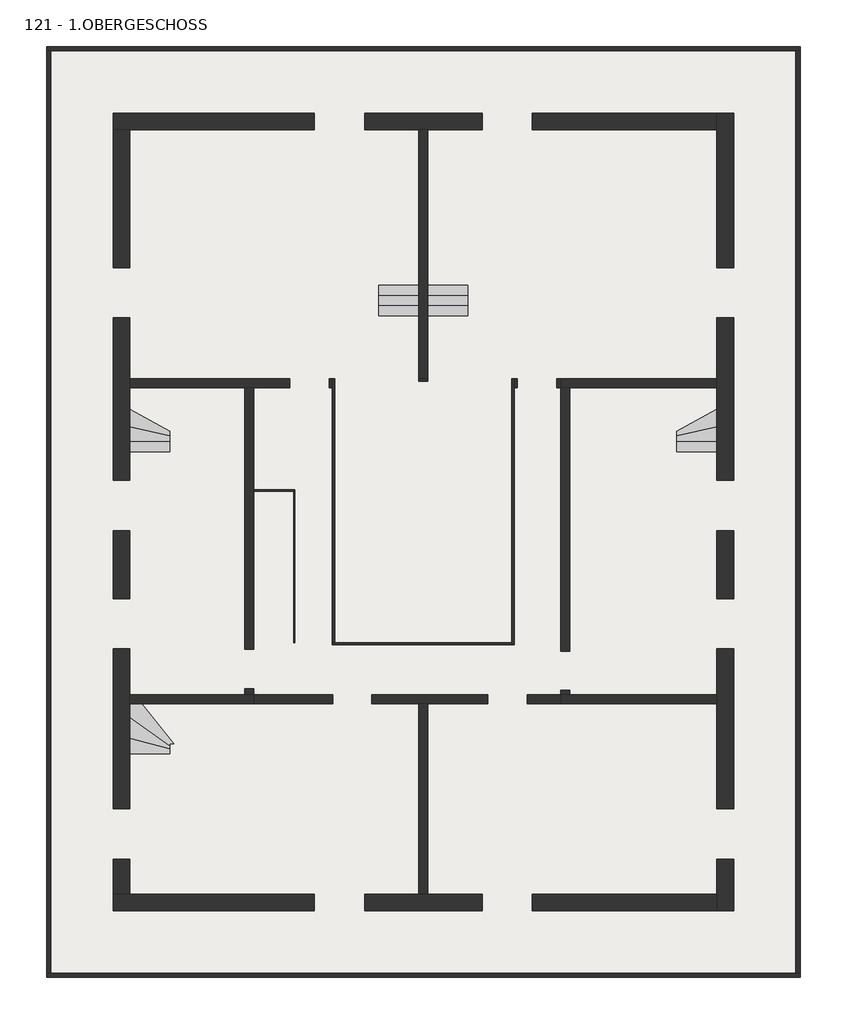
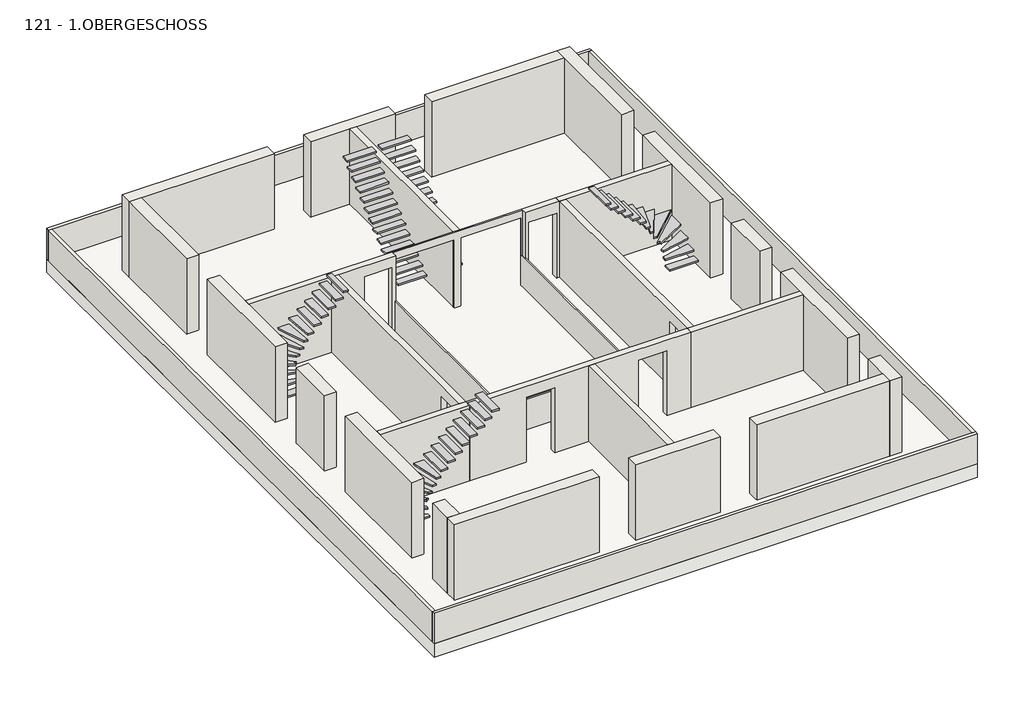
# One storey: 24 walls, 10 stairs, 1 slab.
# Revit data of these elements (continued)
# Project information
#   Organization Name = "Organization Name"
#   Organization Description = "Organization Description"
#   Building Name = "Building Name"
#   IfcOrganization = "KURIARCHITEKTEN"
#   IfcApplicationVersion = "2023.1"
#   IfcApplicationName = "Allplan"
#   IfcSite GUID = "3xMs$kp1n46ejeur8tozco"
#   IfcBuilding GUID = "0i8UyhEYT3nv9HLlo1H2X7"
#   IfcProject GUID = "2x1YFttxr4OvBiL8xtaqeA"
#   NameOverride = "GEBÄUDE 1"
#   Project Issue Date = "Issue Date"
#   Project Status = "Project Status"
#   Client Name = "Client Name"
#   Project Address = "Enter address here\nAddress Line 2"
#   Project Name = "Project Name"
#   Project Number = "Project Number"
# Type "Holzdecke 176 : Holzdecke 176"
#   Abrechnungsart = "m²"
#   Allright_Bauteil_ID = "0113De 0783954357"
#   Bezeichnung = "Holzdecke"
#   Codetext = "D-HOLZBALKEN1\\"
#   Gewerk = "Zimmer- und Holzbauarbeiten"
#   Material = "Holz"
#   Objektname = "Brettstapeldecke"
#   NameOverride = "Holzdecke"
#   Reference = "Holzdecke"
#   Status = "NEW"
#   PitchAngle = 0.00°
#   ThermalTransmittance = 0.0000 BTU/(h·ft²·°F)
#   2D Interaktion = yes
#   Combustible = no
#   Compartmentation = no
#   IsExternal = no
#   LoadBearing = yes
# Type "  97010 :   97010"
#   Abrechnungsart = "St"
#   Allright_Bauteil_ID = "0121Tre0785086959"
#   Material = "Stahlbeton"
#   Objektname = "Treppe"
#   NameOverride = " "
#   ThermalTransmittance = 0.0000 BTU/(h·ft²·°F)
#   NosingLength = 0.000 m
#   NumberOfRiser = 14
#   NumberOfTreads = 14
#   RiserHeight = 2.000 m
#   TreadLength = 2.300 m
#   IsExternal = no
#   FireExit = no
#   HandicapAccessible = no
#   HasNonSkidSurface = no
# Type "  97882 :   97882"
#   Abrechnungsart = "St"
#   Allright_Bauteil_ID = "0121Tre0785065280"
#   Codetext = "TR-MASSIV-GER\\"
#   Material = "Stahlbeton"
#   Objektname = "Treppe"
#   NameOverride = " "
#   Reference = "STB-Treppe"
#   ThermalTransmittance = 0.0000 BTU/(h·ft²·°F)
#   NosingLength = 0.000 m
#   NumberOfRiser = 14
#   NumberOfTreads = 13
#   RiserHeight = 2.021 m
#   TreadLength = 2.300 m
#   IsExternal = no
#   FireExit = no
#   HandicapAccessible = no
#   HasNonSkidSurface = no
# Type "  98300 :   98300"
#   Abrechnungsart = "St"
#   Allright_Bauteil_ID = "0121Tre0785065278"
#   Codetext = "TR-MASSIV-GER\\"
#   Material = "Stahlbeton"
#   Objektname = "Treppe"
#   NameOverride = " "
#   Reference = "STB-Treppe"
#   ThermalTransmittance = 0.0000 BTU/(h·ft²·°F)
#   NosingLength = 0.000 m
#   NumberOfRiser = 14
#   NumberOfTreads = 13
#   RiserHeight = 2.021 m
#   TreadLength = 2.300 m
#   IsExternal = no
#   FireExit = no
#   HandicapAccessible = no
#   HasNonSkidSurface = no
# Type "  98728 :   98728"
#   Abrechnungsart = "St"
#   Allright_Bauteil_ID = "0121Tre0785070507"
#   Material = "Stahlbeton"
#   Objektname = "Treppe"
#   NameOverride = " "
#   ThermalTransmittance = 0.0000 BTU/(h·ft²·°F)
#   NosingLength = 0.000 m
#   NumberOfRiser = 14
#   NumberOfTreads = 13
#   RiserHeight = 2.021 m
#   TreadLength = 2.300 m
#   IsExternal = no
#   FireExit = no
#   HandicapAccessible = no
#   HasNonSkidSurface = no
# Type "  99154 :   99154"
#   Abrechnungsart = "St"
#   Allright_Bauteil_ID = "0121Tre0785070829"
#   Material = "Stahlbeton"
#   Objektname = "Treppe"
#   NameOverride = " "
#   ThermalTransmittance = 0.0000 BTU/(h·ft²·°F)
#   NosingLength = 0.000 m
#   NumberOfRiser = 14
#   NumberOfTreads = 13
#   RiserHeight = 2.021 m
#   TreadLength = 2.300 m
#   IsExternal = no
#   FireExit = no
#   HandicapAccessible = no
#   HasNonSkidSurface = no
# Type "  149542 :   149542"
#   Abrechnungsart = "St"
#   Allright_Bauteil_ID = "0131Tre0659044515"
#   Material = "Stahlbeton"
#   Objektname = "Treppe"
#   NameOverride = " "
#   ThermalTransmittance = 0.0000 BTU/(h·ft²·°F)
#   NosingLength = 0.000 m
#   NumberOfRiser = 14
#   NumberOfTreads = 14
#   RiserHeight = 2.000 m
#   TreadLength = 2.300 m
#   IsExternal = no
#   FireExit = no
#   HandicapAccessible = no
#   HasNonSkidSurface = no
# Type "  150414 :   150414"
#   Abrechnungsart = "St"
#   Allright_Bauteil_ID = "0131Tre0659044575"
#   Codetext = "TR-MASSIV-GER\\"
#   Material = "Stahlbeton"
#   Objektname = "Treppe"
#   NameOverride = " "
#   Reference = "STB-Treppe"
#   ThermalTransmittance = 0.0000 BTU/(h·ft²·°F)
#   NosingLength = 0.000 m
#   NumberOfRiser = 14
#   NumberOfTreads = 13
#   RiserHeight = 2.021 m
#   TreadLength = 2.300 m
#   IsExternal = no
#   FireExit = no
#   HandicapAccessible = no
#   HasNonSkidSurface = no
# Type "  150832 :   150832"
#   Abrechnungsart = "St"
#   Allright_Bauteil_ID = "0131Tre0659044593"
#   Codetext = "TR-MASSIV-GER\\"
#   Material = "Stahlbeton"
#   Objektname = "Treppe"
#   NameOverride = " "
#   Reference = "STB-Treppe"
#   ThermalTransmittance = 0.0000 BTU/(h·ft²·°F)
#   NosingLength = 0.000 m
#   NumberOfRiser = 14
#   NumberOfTreads = 13
#   RiserHeight = 2.021 m
#   TreadLength = 2.300 m
#   IsExternal = no
#   FireExit = no
#   HandicapAccessible = no
#   HasNonSkidSurface = no
# Type "  151260 :   151260"
#   Abrechnungsart = "St"
#   Allright_Bauteil_ID = "0131Tre0659044533"
#   Material = "Stahlbeton"
#   Objektname = "Treppe"
#   NameOverride = " "
#   ThermalTransmittance = 0.0000 BTU/(h·ft²·°F)
#   NosingLength = 0.000 m
#   NumberOfRiser = 14
#   NumberOfTreads = 13
#   RiserHeight = 2.021 m
#   TreadLength = 2.300 m
#   IsExternal = no
#   FireExit = no
#   HandicapAccessible = no
#   HasNonSkidSurface = no
# Type "  151686 :   151686"
#   Abrechnungsart = "St"
#   Allright_Bauteil_ID = "0131Tre0659044570"
#   Material = "Stahlbeton"
#   Objektname = "Treppe"
#   NameOverride = " "
#   ThermalTransmittance = 0.0000 BTU/(h·ft²·°F)
#   NosingLength = 0.000 m
#   NumberOfRiser = 14
#   NumberOfTreads = 13
#   RiserHeight = 2.021 m
#   TreadLength = 2.300 m
#   IsExternal = no
#   FireExit = no
#   HandicapAccessible = no
#   HasNonSkidSurface = no
# Type " :1152"
#   Layers, outside or top first: 0.380 m "holzschalung" (function 1)
# Type " :1161"
#   Layers, outside or top first: 0.380 m "holzschalung" (function 1)
# Type " :1164"
#   Layers, outside or top first: 0.380 m "holzschalung" (function 1)
# Type " :1165"
#   Layers, outside or top first: 0.380 m "holzschalung" (function 1)
# Type " :1166"
#   Layers, outside or top first: 0.050 m "glas" (function 1)
# Type "Holzwand:1150"
#   ThermalTransmittance = 0.0000 BTU/(h·ft²·°F)
#   Combustible = no
#   Compartmentation = no
#   Layers, outside or top first: 0.200 m "holzschalung" (function 1)
# Type "Holzwand:1151"
#   ThermalTransmittance = 0.0000 BTU/(h·ft²·°F)
#   Combustible = no
#   Compartmentation = no
#   Layers, outside or top first: 0.200 m "holzschalung" (function 1)
# Type "Holzwand:1153"
#   ThermalTransmittance = 0.0000 BTU/(h·ft²·°F)
#   Combustible = no
#   Compartmentation = no
#   Layers, outside or top first: 0.200 m "holzschalung" (function 1)
# Type "Holzwand:1154"
#   ThermalTransmittance = 0.0000 BTU/(h·ft²·°F)
#   Combustible = no
#   Compartmentation = no
#   Layers, outside or top first: 0.030 m "holzschalung" (function 1)
# Type "Holzwand:1155"
#   ThermalTransmittance = 0.0000 BTU/(h·ft²·°F)
#   Combustible = no
#   Compartmentation = no
#   Layers, outside or top first: 0.030 m "holzschalung" (function 1)
# Type "Holzwand:1156"
#   ThermalTransmittance = 0.0000 BTU/(h·ft²·°F)
#   Combustible = no
#   Compartmentation = no
#   Layers, outside or top first: 0.200 m "holzschalung" (function 1)
# Type "Holzwand:1157"
#   ThermalTransmittance = 0.0000 BTU/(h·ft²·°F)
#   Combustible = no
#   Compartmentation = no
#   Layers, outside or top first: 0.200 m "holzschalung" (function 1)
# Type "Holzwand:1158"
#   ThermalTransmittance = 0.0000 BTU/(h·ft²·°F)
#   Combustible = no
#   Compartmentation = no
#   Layers, outside or top first: 0.200 m "holzschalung" (function 1)
# Type "Holzwand:1159"
#   ThermalTransmittance = 0.0000 BTU/(h·ft²·°F)
#   Combustible = no
#   Compartmentation = no
#   Layers, outside or top first: 0.200 m "holzschalung" (function 1)
# Type "Holzwand:1160"
#   ThermalTransmittance = 0.0000 BTU/(h·ft²·°F)
#   Combustible = no
#   Compartmentation = no
#   Layers, outside or top first: 0.200 m "holzschalung" (function 1)
# Type "Holzwand:1162"
#   ThermalTransmittance = 0.0000 BTU/(h·ft²·°F)
#   Combustible = no
#   Compartmentation = no
#   Layers, outside or top first: 0.200 m "holzschalung" (function 1)
# Type "Holzwand:1163"
#   ThermalTransmittance = 0.0000 BTU/(h·ft²·°F)
#   Combustible = no
#   Compartmentation = no
#   Layers, outside or top first: 0.200 m "holzschalung" (function 1)
# Type " :1167"
#   Layers, outside or top first: 0.050 m "holzschalung" (function 1)
# Type " :1168"
#   Layers, outside or top first: 0.050 m "holzschalung" (function 1)
# Type " :1169"
#   Layers, outside or top first: 0.050 m "holzschalung" (function 1)
# Type "Holzwand:1170"
#   ThermalTransmittance = 0.0000 BTU/(h·ft²·°F)
#   Combustible = no
#   Compartmentation = no
#   Layers, outside or top first: 0.100 m "pv - panel anthrazit" (function 1)
# Type "Holzwand:1171"
#   ThermalTransmittance = 0.0000 BTU/(h·ft²·°F)
#   Combustible = no
#   Compartmentation = no
#   Layers, outside or top first: 0.100 m "pv - panel anthrazit" (function 1)
# Type "Holzwand:1172"
#   ThermalTransmittance = 0.0000 BTU/(h·ft²·°F)
#   Combustible = no
#   Compartmentation = no
#   Layers, outside or top first: 0.100 m "pv - panel anthrazit" (function 1)
# Type "Holzwand:1173"
#   ThermalTransmittance = 0.0000 BTU/(h·ft²·°F)
#   Combustible = no
#   Compartmentation = no
#   Layers, outside or top first: 0.100 m "pv - panel anthrazit" (function 1)
# Element 1 (IfcSlab, "Holzdecke 176 : Holzdecke 176")
#   IFC Predefined Type = "FLOOR"
#   Export to IFC As = "ifcslab"
#   IfcGUID = "1_9Us2eVX4OuIZjhNyqdxW"
#   Phase Created = New Construction
#   Materials on its faces: "holzschalung"
# Element 2 (IfcStair, "  97010 :   97010")
#   IFC Predefined Type = "NOTDEFINED"
#   Export to IFC As = "ifcstair"
#   IfcGUID = "2ccaodaeb6QgHPV1d4NBnA"
#   Phase Created = New Construction
#   Materials on its faces: "weiss"
# Element 3 (IfcStair, "  97882 :   97882")
#   IFC Predefined Type = "STRAIGHT_RUN_STAIR"
#   Export to IFC As = "ifcstair"
#   IfcGUID = "1nghyUHoH9yBc_lxkBTUjw"
#   Phase Created = New Construction
#   Materials on its faces: "weiss"
# Element 4 (IfcStair, "  98300 :   98300")
#   IFC Predefined Type = "STRAIGHT_RUN_STAIR"
#   Export to IFC As = "ifcstair"
#   IfcGUID = "2AC_Gmfhz1LvYwUyPOxWan"
#   Phase Created = New Construction
#   Materials on its faces: "weiss"
# Element 5 (IfcStair, "  98728 :   98728")
#   IFC Predefined Type = "NOTDEFINED"
#   Export to IFC As = "ifcstair"
#   IfcGUID = "04Edcgbk9CPwWYiYhycXFf"
#   Phase Created = New Construction
#   Materials on its faces: "weiss"
# Element 6 (IfcStair, "  99154 :   99154")
#   IFC Predefined Type = "NOTDEFINED"
#   Export to IFC As = "ifcstair"
#   IfcGUID = "1azVXxNdn2POY9VYN93ccY"
#   Phase Created = New Construction
#   Materials on its faces: "weiss"
# Element 7 (IfcStair, "  149542 :   149542")
#   IFC Predefined Type = "NOTDEFINED"
#   Export to IFC As = "ifcstair"
#   IfcGUID = "1sH4rJKnLAFOtHPnXrLkif"
#   Phase Created = New Construction
#   Materials on its faces: "weiss"
# Element 8 (IfcStair, "  150414 :   150414")
#   IFC Predefined Type = "STRAIGHT_RUN_STAIR"
#   Export to IFC As = "ifcstair"
#   IfcGUID = "3fdccs_Mj1YAyFFpBc3gyk"
#   Phase Created = New Construction
#   Materials on its faces: "weiss"
# Element 9 (IfcStair, "  150832 :   150832")
#   IFC Predefined Type = "STRAIGHT_RUN_STAIR"
#   Export to IFC As = "ifcstair"
#   IfcGUID = "2szmEZdbD3KBDvfX1Sa6Vh"
#   Phase Created = New Construction
#   Materials on its faces: "weiss"
# Element 10 (IfcStair, "  151260 :   151260")
#   IFC Predefined Type = "NOTDEFINED"
#   Export to IFC As = "ifcstair"
#   IfcGUID = "1YKyaFTbr8YR41yGjubBsl"
#   Phase Created = New Construction
#   Materials on its faces: "weiss"
# Element 11 (IfcStair, "  151686 :   151686")
#   IFC Predefined Type = "NOTDEFINED"
#   Export to IFC As = "ifcstair"
#   IfcGUID = "2KPGRYHzzCygzBebAeLtPz"
#   Phase Created = New Construction
#   Materials on its faces: "weiss"
# Element 12 (IfcWall, " :1152")
#   Export to IFC As = "ifcwall"
#   IfcGUID = "2CeDj8YZTCPx$yj4WDVOez"
#   NameOverride = " "
#   Abrechnungsart = "m³"
#   Allright_Bauteil_ID = "0121HWa0785064286"
#   Layer #1:Object Layer Attributes #1:Abrechnungsart = "m²"
#   Layer #1:Object Layer Attributes #1:Allright_Bauteil_ID = "0121Wa 0785064367"
#   Layer #1:Object Layer Attributes #1:Gewerk = "Zimmer- und Holzbauarbeiten"
#   Layer #1:Object Layer Attributes #1:Material = "k.Ausw."
#   Layer #1:Object Layer Attributes #1:Objektname = "Wand"
#   Layer #1:Object Layer Attributes #1:Status = "Neubau"
#   MEP Wandtyp = "HO-WA-HSW\\"
#   Objektname = "Gesamtwand"
#   built-in parameter 1001111 = 0.505 m
#   Top Offset = 0.000 m
#   Base Offset = 0.505 m
#   Unconnected Height = 2.500 m
#   wall height = 2.500 m
#   Layer #1:Object Layer Attributes #1:2D Interaktion = yes
#   Phase Created = New Construction
#   Base Constraint = 121 - 1.OBERGESCHOSS
#   Materials on its faces: "holzschalung"
# Element 13 (IfcWall, " :1161")
#   Export to IFC As = "ifcwall"
#   IfcGUID = "2TnImcbz91shb3jN7Wgb8B"
#   NameOverride = " "
#   Abrechnungsart = "m³"
#   Allright_Bauteil_ID = "0121HWa0785064349"
#   Layer #1:Object Layer Attributes #1:Abrechnungsart = "m²"
#   Layer #1:Object Layer Attributes #1:Allright_Bauteil_ID = "0121Wa 0785064397"
#   Layer #1:Object Layer Attributes #1:Gewerk = "Zimmer- und Holzbauarbeiten"
#   Layer #1:Object Layer Attributes #1:Material = "k.Ausw."
#   Layer #1:Object Layer Attributes #1:Objektname = "Wand"
#   Layer #1:Object Layer Attributes #1:Status = "Neubau"
#   MEP Wandtyp = "HO-WA-HSW\\"
#   Objektname = "Gesamtwand"
#   built-in parameter 1001111 = 0.505 m
#   Top Offset = 0.000 m
#   Base Offset = 0.505 m
#   Unconnected Height = 2.500 m
#   wall height = 2.500 m
#   Layer #1:Object Layer Attributes #1:2D Interaktion = yes
#   Phase Created = New Construction
#   Base Constraint = 121 - 1.OBERGESCHOSS
#   Materials on its faces: "holzschalung"
# Element 14 (IfcWall, " :1164")
#   Export to IFC As = "ifcwall"
#   IfcGUID = "1tWRh4hxLAdASVw4VNE3to"
#   NameOverride = " "
#   Abrechnungsart = "m³"
#   Allright_Bauteil_ID = "0121HWa0785092952"
#   Layer #1:Object Layer Attributes #1:Abrechnungsart = "m²"
#   Layer #1:Object Layer Attributes #1:Allright_Bauteil_ID = "0121Wa 0785092986"
#   Layer #1:Object Layer Attributes #1:Gewerk = "Zimmer- und Holzbauarbeiten"
#   Layer #1:Object Layer Attributes #1:Material = "k.Ausw."
#   Layer #1:Object Layer Attributes #1:Objektname = "Wand"
#   Layer #1:Object Layer Attributes #1:Status = "Neubau"
#   MEP Wandtyp = "HO-WA-HSW\\"
#   Objektname = "Gesamtwand"
#   built-in parameter 1001111 = 0.505 m
#   Top Offset = 0.000 m
#   Base Offset = 0.505 m
#   Unconnected Height = 2.500 m
#   wall height = 2.500 m
#   Layer #1:Object Layer Attributes #1:2D Interaktion = yes
#   Phase Created = New Construction
#   Base Constraint = 121 - 1.OBERGESCHOSS
#   Materials on its faces: "holzschalung"
# Element 15 (IfcWall, " :1165")
#   Export to IFC As = "ifcwall"
#   IfcGUID = "1HE73MTmDEEBf4AV7ughZ8"
#   NameOverride = " "
#   Abrechnungsart = "m³"
#   Allright_Bauteil_ID = "0121HWa0785097898"
#   Layer #1:Object Layer Attributes #1:Abrechnungsart = "m²"
#   Layer #1:Object Layer Attributes #1:Allright_Bauteil_ID = "0121Wa 0785097934"
#   Layer #1:Object Layer Attributes #1:Gewerk = "Zimmer- und Holzbauarbeiten"
#   Layer #1:Object Layer Attributes #1:Material = "k.Ausw."
#   Layer #1:Object Layer Attributes #1:Objektname = "Wand"
#   Layer #1:Object Layer Attributes #1:Status = "Neubau"
#   MEP Wandtyp = "HO-WA-HSW\\"
#   Objektname = "Gesamtwand"
#   built-in parameter 1001111 = 0.505 m
#   Top Offset = 0.000 m
#   Base Offset = 0.505 m
#   Unconnected Height = 2.500 m
#   wall height = 2.500 m
#   Layer #1:Object Layer Attributes #1:2D Interaktion = yes
#   Phase Created = New Construction
#   Base Constraint = 121 - 1.OBERGESCHOSS
#   Materials on its faces: "holzschalung"
# Element 16 (IfcWall, " :1166")
#   Export to IFC As = "ifcwall"
#   IfcGUID = "0t2qqx1kvDZPNPdKl4bfzP"
#   NameOverride = " "
#   Abrechnungsart = "m³"
#   Allright_Bauteil_ID = "0121HWa0785064296"
#   Layer #1:Object Layer Attributes #1:Abrechnungsart = "m²"
#   Layer #1:Object Layer Attributes #1:Allright_Bauteil_ID = "0121Wa 0785064386"
#   Layer #1:Object Layer Attributes #1:Gewerk = "Zimmer- und Holzbauarbeiten"
#   Layer #1:Object Layer Attributes #1:Material = "k.Ausw."
#   Layer #1:Object Layer Attributes #1:Objektname = "Wand"
#   Layer #1:Object Layer Attributes #1:Status = "Neubau"
#   MEP Wandtyp = "HO-WA-HSW\\"
#   Objektname = "Gesamtwand"
#   built-in parameter 1001111 = 0.505 m
#   Top Offset = 0.000 m
#   Base Offset = 0.505 m
#   Unconnected Height = 2.500 m
#   wall height = 2.500 m
#   Layer #1:Object Layer Attributes #1:2D Interaktion = yes
#   Phase Created = New Construction
#   Base Constraint = 121 - 1.OBERGESCHOSS
#   Materials on its faces: "glas"
# Element 17 (IfcWall, "Holzwand:1150")
#   Export to IFC As = "ifcwall"
#   IfcGUID = "3nZ5Mon9nBjwoRgvyoor9a"
#   NameOverride = "Holzwand"
#   Abrechnungsart = "St"
#   Allright_Bauteil_ID = "0121HWa0785065367"
#   Bezeichnung = "Holzwand"
#   Layer #1:Object Layer Attributes #1:Abrechnungsart = "m²"
#   Layer #1:Object Layer Attributes #1:Allright_Bauteil_ID = "0121Wa 0785065369"
#   Layer #1:Object Layer Attributes #1:Bezeichnung = "Holzwand"
#   Layer #1:Object Layer Attributes #1:Codetext = "HO-WI-HSW\\"
#   Layer #1:Object Layer Attributes #1:Gewerk = "Zimmer- und Holzbauarbeiten"
#   Layer #1:Object Layer Attributes #1:Material = "Holz"
#   Layer #1:Object Layer Attributes #1:Objektname = "Wand"
#   Layer #1:Object Layer Attributes #1:Reference = "Holzwand"
#   Layer #1:Object Layer Attributes #1:Status = "Neubau"
#   MEP Wandtyp = "HO-WA-HSW\\"
#   Objektname = "Gesamtwand"
#   Reference = "Holzwand"
#   Status = "NEW"
#   built-in parameter 1001111 = 0.505 m
#   Top Offset = 0.000 m
#   Base Offset = 0.505 m
#   Unconnected Height = 2.500 m
#   wall height = 2.500 m
#   Layer #1:Object Layer Attributes #1:U-Wert = 0
#   Layer #1:Object Layer Attributes #1:2D Interaktion = yes
#   Layer #1:Object Layer Attributes #1:Außenbauteil = no
#   Layer #1:Object Layer Attributes #1:Brandabschnittsdefinierendes Bauteil = no
#   Layer #1:Object Layer Attributes #1:Brennbares Material = no
#   Layer #1:Object Layer Attributes #1:Raumhohe Wand = yes
#   Layer #1:Object Layer Attributes #1:Tragendes Bauteil = yes
#   ExtendToStructure = yes
#   IsExternal = no
#   LoadBearing = yes
#   Phase Created = New Construction
#   Base Constraint = 121 - 1.OBERGESCHOSS
#   Materials on its faces: "holzschalung"
# Element 18 (IfcWall, "Holzwand:1151")
#   Export to IFC As = "ifcwall"
#   IfcGUID = "3jE1E$NFj7vAP$vn70kdrt"
#   NameOverride = "Holzwand"
#   Abrechnungsart = "St"
#   Allright_Bauteil_ID = "0121HWa0785066899"
#   Bezeichnung = "Holzwand"
#   Layer #1:Object Layer Attributes #1:Abrechnungsart = "m²"
#   Layer #1:Object Layer Attributes #1:Allright_Bauteil_ID = "0121Wa 0785066901"
#   Layer #1:Object Layer Attributes #1:Bezeichnung = "Holzwand"
#   Layer #1:Object Layer Attributes #1:Codetext = "HO-WI-HSW\\"
#   Layer #1:Object Layer Attributes #1:Gewerk = "Zimmer- und Holzbauarbeiten"
#   Layer #1:Object Layer Attributes #1:Material = "Holz"
#   Layer #1:Object Layer Attributes #1:Objektname = "Wand"
#   Layer #1:Object Layer Attributes #1:Reference = "Holzwand"
#   Layer #1:Object Layer Attributes #1:Status = "Neubau"
#   MEP Wandtyp = "HO-WA-HSW\\"
#   Objektname = "Gesamtwand"
#   Reference = "Holzwand"
#   Status = "NEW"
#   built-in parameter 1001111 = 0.505 m
#   Top Offset = 0.000 m
#   Base Offset = 0.505 m
#   Unconnected Height = 2.500 m
#   wall height = 2.500 m
#   Layer #1:Object Layer Attributes #1:U-Wert = 0
#   Layer #1:Object Layer Attributes #1:2D Interaktion = yes
#   Layer #1:Object Layer Attributes #1:Außenbauteil = no
#   Layer #1:Object Layer Attributes #1:Brandabschnittsdefinierendes Bauteil = no
#   Layer #1:Object Layer Attributes #1:Brennbares Material = no
#   Layer #1:Object Layer Attributes #1:Raumhohe Wand = yes
#   Layer #1:Object Layer Attributes #1:Tragendes Bauteil = yes
#   ExtendToStructure = yes
#   IsExternal = no
#   LoadBearing = yes
#   Phase Created = New Construction
#   Base Constraint = 121 - 1.OBERGESCHOSS
#   Materials on its faces: "holzschalung"
# Element 19 (IfcWall, "Holzwand:1153")
#   Export to IFC As = "ifcwall"
#   IfcGUID = "1Zhxv5EALB9e6_$pCtUEXg"
#   NameOverride = "Holzwand"
#   Abrechnungsart = "St"
#   Allright_Bauteil_ID = "0121HWa0785065540"
#   Bezeichnung = "Holzwand"
#   Layer #1:Object Layer Attributes #1:Abrechnungsart = "m²"
#   Layer #1:Object Layer Attributes #1:Allright_Bauteil_ID = "0121Wa 0785065541"
#   Layer #1:Object Layer Attributes #1:Bezeichnung = "Holzwand"
#   Layer #1:Object Layer Attributes #1:Codetext = "HO-WI-HSW\\"
#   Layer #1:Object Layer Attributes #1:Gewerk = "Zimmer- und Holzbauarbeiten"
#   Layer #1:Object Layer Attributes #1:Material = "Holz"
#   Layer #1:Object Layer Attributes #1:Objektname = "Wand"
#   Layer #1:Object Layer Attributes #1:Reference = "Holzwand"
#   Layer #1:Object Layer Attributes #1:Status = "Neubau"
#   MEP Wandtyp = "HO-WA-HSW\\"
#   Objektname = "Gesamtwand"
#   Reference = "Holzwand"
#   Status = "NEW"
#   built-in parameter 1001111 = 0.505 m
#   Top Offset = 0.000 m
#   Base Offset = 0.505 m
#   Unconnected Height = 2.500 m
#   wall height = 2.500 m
#   Layer #1:Object Layer Attributes #1:U-Wert = 0
#   Layer #1:Object Layer Attributes #1:2D Interaktion = yes
#   Layer #1:Object Layer Attributes #1:Außenbauteil = no
#   Layer #1:Object Layer Attributes #1:Brandabschnittsdefinierendes Bauteil = no
#   Layer #1:Object Layer Attributes #1:Brennbares Material = no
#   Layer #1:Object Layer Attributes #1:Raumhohe Wand = yes
#   Layer #1:Object Layer Attributes #1:Tragendes Bauteil = yes
#   ExtendToStructure = yes
#   IsExternal = no
#   LoadBearing = yes
#   Phase Created = New Construction
#   Base Constraint = 121 - 1.OBERGESCHOSS
#   Materials on its faces: "holzschalung"
# Element 20 (IfcWall, "Holzwand:1154")
#   Export to IFC As = "ifcwall"
#   IfcGUID = "2MsVq3EJn0K8wHdQ6uoxnd"
#   NameOverride = "Holzwand"
#   Abrechnungsart = "St"
#   Allright_Bauteil_ID = "0121HWa0785067355"
#   Bezeichnung = "Holzwand"
#   Layer #1:Object Layer Attributes #1:Abrechnungsart = "m²"
#   Layer #1:Object Layer Attributes #1:Allright_Bauteil_ID = "0121Wa 0785067356"
#   Layer #1:Object Layer Attributes #1:Codetext = "HO-WI-HSW\\"
#   Layer #1:Object Layer Attributes #1:Gewerk = "Zimmer- und Holzbauarbeiten"
#   Layer #1:Object Layer Attributes #1:Material = "Holz"
#   Layer #1:Object Layer Attributes #1:Objektname = "Wand"
#   Layer #1:Object Layer Attributes #1:Reference = "Holzwand"
#   Layer #1:Object Layer Attributes #1:Status = "Neubau"
#   MEP Wandtyp = "HO-WA-HSW\\"
#   Objektname = "Gesamtwand"
#   Reference = "Holzwand"
#   Status = "NEW"
#   built-in parameter 1001111 = 0.505 m
#   Top Offset = 0.000 m
#   Base Offset = 0.505 m
#   Unconnected Height = 1.000 m
#   wall height = 1.000 m
#   Layer #1:Object Layer Attributes #1:U-Wert = 0
#   Layer #1:Object Layer Attributes #1:2D Interaktion = yes
#   Layer #1:Object Layer Attributes #1:Außenbauteil = no
#   Layer #1:Object Layer Attributes #1:Brandabschnittsdefinierendes Bauteil = no
#   Layer #1:Object Layer Attributes #1:Brennbares Material = no
#   Layer #1:Object Layer Attributes #1:Raumhohe Wand = yes
#   ExtendToStructure = yes
#   IsExternal = no
#   LoadBearing = yes
#   Phase Created = New Construction
#   Base Constraint = 121 - 1.OBERGESCHOSS
#   Materials on its faces: "holzschalung"
# Element 21 (IfcWall, "Holzwand:1155")
#   Export to IFC As = "ifcwall"
#   IfcGUID = "1F_ySrDsP9oP3MqXymSTVO"
#   NameOverride = "Holzwand"
#   Abrechnungsart = "St"
#   Allright_Bauteil_ID = "0121HWa0785067347"
#   Bezeichnung = "Holzwand"
#   Layer #1:Object Layer Attributes #1:Abrechnungsart = "m²"
#   Layer #1:Object Layer Attributes #1:Allright_Bauteil_ID = "0121Wa 0785067348"
#   Layer #1:Object Layer Attributes #1:Codetext = "HO-WI-HSW\\"
#   Layer #1:Object Layer Attributes #1:Gewerk = "Zimmer- und Holzbauarbeiten"
#   Layer #1:Object Layer Attributes #1:Material = "Holz"
#   Layer #1:Object Layer Attributes #1:Objektname = "Wand"
#   Layer #1:Object Layer Attributes #1:Reference = "Holzwand"
#   Layer #1:Object Layer Attributes #1:Status = "Neubau"
#   MEP Wandtyp = "HO-WA-HSW\\"
#   Objektname = "Gesamtwand"
#   Reference = "Holzwand"
#   Status = "NEW"
#   built-in parameter 1001111 = 0.505 m
#   Top Offset = 0.000 m
#   Base Offset = 0.505 m
#   Unconnected Height = 1.000 m
#   wall height = 1.000 m
#   Layer #1:Object Layer Attributes #1:U-Wert = 0
#   Layer #1:Object Layer Attributes #1:2D Interaktion = yes
#   Layer #1:Object Layer Attributes #1:Außenbauteil = no
#   Layer #1:Object Layer Attributes #1:Brandabschnittsdefinierendes Bauteil = no
#   Layer #1:Object Layer Attributes #1:Brennbares Material = no
#   Layer #1:Object Layer Attributes #1:Raumhohe Wand = yes
#   ExtendToStructure = yes
#   IsExternal = no
#   LoadBearing = yes
#   Phase Created = New Construction
#   Base Constraint = 121 - 1.OBERGESCHOSS
#   Materials on its faces: "holzschalung"
# Element 22 (IfcWall, "Holzwand:1156")
#   Export to IFC As = "ifcwall"
#   IfcGUID = "0gtwZwppj1pObqyI7HY41_"
#   NameOverride = "Holzwand"
#   Abrechnungsart = "St"
#   Allright_Bauteil_ID = "0121HWa0785064323"
#   Bezeichnung = "Holzwand"
#   Layer #1:Object Layer Attributes #1:Abrechnungsart = "m²"
#   Layer #1:Object Layer Attributes #1:Allright_Bauteil_ID = "0121Wa 0785064369"
#   Layer #1:Object Layer Attributes #1:Bezeichnung = "Holzwand"
#   Layer #1:Object Layer Attributes #1:Codetext = "HO-WI-HSW\\"
#   Layer #1:Object Layer Attributes #1:Gewerk = "Zimmer- und Holzbauarbeiten"
#   Layer #1:Object Layer Attributes #1:Material = "Holz"
#   Layer #1:Object Layer Attributes #1:Objektname = "Wand"
#   Layer #1:Object Layer Attributes #1:Reference = "Holzwand"
#   Layer #1:Object Layer Attributes #1:Status = "Neubau"
#   MEP Wandtyp = "HO-WA-HSW\\"
#   Objektname = "Gesamtwand"
#   Reference = "Holzwand"
#   Status = "NEW"
#   built-in parameter 1001111 = 0.505 m
#   Top Offset = 0.000 m
#   Base Offset = 0.505 m
#   Unconnected Height = 2.500 m
#   wall height = 2.500 m
#   Layer #1:Object Layer Attributes #1:U-Wert = 0
#   Layer #1:Object Layer Attributes #1:2D Interaktion = yes
#   Layer #1:Object Layer Attributes #1:Außenbauteil = no
#   Layer #1:Object Layer Attributes #1:Brandabschnittsdefinierendes Bauteil = no
#   Layer #1:Object Layer Attributes #1:Brennbares Material = no
#   Layer #1:Object Layer Attributes #1:Raumhohe Wand = yes
#   Layer #1:Object Layer Attributes #1:Tragendes Bauteil = yes
#   ExtendToStructure = yes
#   IsExternal = no
#   LoadBearing = yes
#   Phase Created = New Construction
#   Base Constraint = 121 - 1.OBERGESCHOSS
#   Materials on its faces: "holzschalung"
# Element 23 (IfcWall, "Holzwand:1157")
#   Export to IFC As = "ifcwall"
#   IfcGUID = "0tY6$O1l121AktLhYSWZjf"
#   NameOverride = "Holzwand"
#   Abrechnungsart = "St"
#   Allright_Bauteil_ID = "0121HWa0785064381"
#   Bezeichnung = "Holzwand"
#   Layer #1:Object Layer Attributes #1:Abrechnungsart = "m²"
#   Layer #1:Object Layer Attributes #1:Allright_Bauteil_ID = "0121Wa 0785064384"
#   Layer #1:Object Layer Attributes #1:Bezeichnung = "Holzwand"
#   Layer #1:Object Layer Attributes #1:Codetext = "HO-WI-HSW\\"
#   Layer #1:Object Layer Attributes #1:Gewerk = "Zimmer- und Holzbauarbeiten"
#   Layer #1:Object Layer Attributes #1:Material = "Holz"
#   Layer #1:Object Layer Attributes #1:Objektname = "Wand"
#   Layer #1:Object Layer Attributes #1:Reference = "Holzwand"
#   Layer #1:Object Layer Attributes #1:Status = "Neubau"
#   MEP Wandtyp = "HO-WA-HSW\\"
#   Objektname = "Gesamtwand"
#   Reference = "Holzwand"
#   Status = "NEW"
#   built-in parameter 1001111 = 0.505 m
#   Top Offset = 0.000 m
#   Base Offset = 0.505 m
#   Unconnected Height = 2.500 m
#   wall height = 2.500 m
#   Layer #1:Object Layer Attributes #1:U-Wert = 0
#   Layer #1:Object Layer Attributes #1:2D Interaktion = yes
#   Layer #1:Object Layer Attributes #1:Außenbauteil = no
#   Layer #1:Object Layer Attributes #1:Brandabschnittsdefinierendes Bauteil = no
#   Layer #1:Object Layer Attributes #1:Brennbares Material = no
#   Layer #1:Object Layer Attributes #1:Raumhohe Wand = yes
#   Layer #1:Object Layer Attributes #1:Tragendes Bauteil = yes
#   ExtendToStructure = yes
#   IsExternal = no
#   LoadBearing = yes
#   Phase Created = New Construction
#   Base Constraint = 121 - 1.OBERGESCHOSS
#   Materials on its faces: "holzschalung"
# Element 24 (IfcWall, "Holzwand:1158")
#   Export to IFC As = "ifcwall"
#   IfcGUID = "2Mr8L52dj4iP8MoJTiOa9p"
#   NameOverride = "Holzwand"
#   Abrechnungsart = "St"
#   Allright_Bauteil_ID = "0121HWa0785069286"
#   Bezeichnung = "Holzwand"
#   Layer #1:Object Layer Attributes #1:Abrechnungsart = "m²"
#   Layer #1:Object Layer Attributes #1:Allright_Bauteil_ID = "0121Wa 0785069294"
#   Layer #1:Object Layer Attributes #1:Bezeichnung = "Holzwand"
#   Layer #1:Object Layer Attributes #1:Codetext = "HO-WI-HSW\\"
#   Layer #1:Object Layer Attributes #1:Gewerk = "Zimmer- und Holzbauarbeiten"
#   Layer #1:Object Layer Attributes #1:Material = "Holz"
#   Layer #1:Object Layer Attributes #1:Objektname = "Wand"
#   Layer #1:Object Layer Attributes #1:Reference = "Holzwand"
#   Layer #1:Object Layer Attributes #1:Status = "Neubau"
#   MEP Wandtyp = "HO-WA-HSW\\"
#   Objektname = "Gesamtwand"
#   Reference = "Holzwand"
#   Status = "NEW"
#   built-in parameter 1001111 = 0.505 m
#   Top Offset = 0.000 m
#   Base Offset = 0.505 m
#   Unconnected Height = 2.500 m
#   wall height = 2.500 m
#   Layer #1:Object Layer Attributes #1:U-Wert = 0
#   Layer #1:Object Layer Attributes #1:2D Interaktion = yes
#   Layer #1:Object Layer Attributes #1:Außenbauteil = no
#   Layer #1:Object Layer Attributes #1:Brandabschnittsdefinierendes Bauteil = no
#   Layer #1:Object Layer Attributes #1:Brennbares Material = no
#   Layer #1:Object Layer Attributes #1:Raumhohe Wand = yes
#   Layer #1:Object Layer Attributes #1:Tragendes Bauteil = yes
#   ExtendToStructure = yes
#   IsExternal = no
#   LoadBearing = yes
#   Phase Created = New Construction
#   Base Constraint = 121 - 1.OBERGESCHOSS
#   Materials on its faces: "holzschalung"
# Element 25 (IfcWall, "Holzwand:1159")
#   Export to IFC As = "ifcwall"
#   IfcGUID = "36leNf4gL9OB_v358ffY76"
#   NameOverride = "Holzwand"
#   Abrechnungsart = "St"
#   Allright_Bauteil_ID = "0121HWa0785064324"
#   Bezeichnung = "Holzwand"
#   Layer #1:Object Layer Attributes #1:Abrechnungsart = "m²"
#   Layer #1:Object Layer Attributes #1:Allright_Bauteil_ID = "0121Wa 0785064395"
#   Layer #1:Object Layer Attributes #1:Bezeichnung = "Holzwand"
#   Layer #1:Object Layer Attributes #1:Codetext = "HO-WI-HSW\\"
#   Layer #1:Object Layer Attributes #1:Gewerk = "Zimmer- und Holzbauarbeiten"
#   Layer #1:Object Layer Attributes #1:Material = "Holz"
#   Layer #1:Object Layer Attributes #1:Objektname = "Wand"
#   Layer #1:Object Layer Attributes #1:Reference = "Holzwand"
#   Layer #1:Object Layer Attributes #1:Status = "Neubau"
#   MEP Wandtyp = "HO-WA-HSW\\"
#   Objektname = "Gesamtwand"
#   Reference = "Holzwand"
#   Status = "NEW"
#   built-in parameter 1001111 = 0.505 m
#   Top Offset = 0.000 m
#   Base Offset = 0.505 m
#   Unconnected Height = 2.500 m
#   wall height = 2.500 m
#   Layer #1:Object Layer Attributes #1:U-Wert = 0
#   Layer #1:Object Layer Attributes #1:2D Interaktion = yes
#   Layer #1:Object Layer Attributes #1:Außenbauteil = no
#   Layer #1:Object Layer Attributes #1:Brandabschnittsdefinierendes Bauteil = no
#   Layer #1:Object Layer Attributes #1:Brennbares Material = no
#   Layer #1:Object Layer Attributes #1:Raumhohe Wand = yes
#   Layer #1:Object Layer Attributes #1:Tragendes Bauteil = yes
#   ExtendToStructure = yes
#   IsExternal = no
#   LoadBearing = yes
#   Phase Created = New Construction
#   Base Constraint = 121 - 1.OBERGESCHOSS
#   Materials on its faces: "holzschalung"
# Element 26 (IfcWall, "Holzwand:1160")
#   Export to IFC As = "ifcwall"
#   IfcGUID = "3kHHpx_NTE_9JnfL3dFkYB"
#   NameOverride = "Holzwand"
#   Abrechnungsart = "St"
#   Allright_Bauteil_ID = "0121HWa0785064389"
#   Bezeichnung = "Holzwand"
#   Layer #1:Object Layer Attributes #1:Abrechnungsart = "m²"
#   Layer #1:Object Layer Attributes #1:Allright_Bauteil_ID = "0121Wa 0785064393"
#   Layer #1:Object Layer Attributes #1:Bezeichnung = "Holzwand"
#   Layer #1:Object Layer Attributes #1:Codetext = "HO-WI-HSW\\"
#   Layer #1:Object Layer Attributes #1:Gewerk = "Zimmer- und Holzbauarbeiten"
#   Layer #1:Object Layer Attributes #1:Material = "Holz"
#   Layer #1:Object Layer Attributes #1:Objektname = "Wand"
#   Layer #1:Object Layer Attributes #1:Reference = "Holzwand"
#   Layer #1:Object Layer Attributes #1:Status = "Neubau"
#   MEP Wandtyp = "HO-WA-HSW\\"
#   Objektname = "Gesamtwand"
#   Reference = "Holzwand"
#   Status = "NEW"
#   built-in parameter 1001111 = 0.505 m
#   Top Offset = 0.000 m
#   Base Offset = 0.505 m
#   Unconnected Height = 2.500 m
#   wall height = 2.500 m
#   Layer #1:Object Layer Attributes #1:U-Wert = 0
#   Layer #1:Object Layer Attributes #1:2D Interaktion = yes
#   Layer #1:Object Layer Attributes #1:Außenbauteil = no
#   Layer #1:Object Layer Attributes #1:Brandabschnittsdefinierendes Bauteil = no
#   Layer #1:Object Layer Attributes #1:Brennbares Material = no
#   Layer #1:Object Layer Attributes #1:Raumhohe Wand = yes
#   Layer #1:Object Layer Attributes #1:Tragendes Bauteil = yes
#   ExtendToStructure = yes
#   IsExternal = no
#   LoadBearing = yes
#   Phase Created = New Construction
#   Base Constraint = 121 - 1.OBERGESCHOSS
#   Materials on its faces: "holzschalung"
# Element 27 (IfcWall, "Holzwand:1162")
#   Export to IFC As = "ifcwall"
#   IfcGUID = "26lQuimMP00PZvPhbBRI2R"
#   NameOverride = "Holzwand"
#   Abrechnungsart = "St"
#   Allright_Bauteil_ID = "0121HWa0785065329"
#   Bezeichnung = "Holzwand"
#   Layer #1:Object Layer Attributes #1:Abrechnungsart = "m²"
#   Layer #1:Object Layer Attributes #1:Allright_Bauteil_ID = "0121Wa 0785065331"
#   Layer #1:Object Layer Attributes #1:Bezeichnung = "Holzwand"
#   Layer #1:Object Layer Attributes #1:Codetext = "HO-WI-HSW\\"
#   Layer #1:Object Layer Attributes #1:Gewerk = "Zimmer- und Holzbauarbeiten"
#   Layer #1:Object Layer Attributes #1:Material = "Holz"
#   Layer #1:Object Layer Attributes #1:Objektname = "Wand"
#   Layer #1:Object Layer Attributes #1:Reference = "Holzwand"
#   Layer #1:Object Layer Attributes #1:Status = "Neubau"
#   MEP Wandtyp = "HO-WA-HSW\\"
#   Objektname = "Gesamtwand"
#   Reference = "Holzwand"
#   Status = "NEW"
#   built-in parameter 1001111 = 0.505 m
#   Top Offset = 0.000 m
#   Base Offset = 0.505 m
#   Unconnected Height = 2.500 m
#   wall height = 2.500 m
#   Layer #1:Object Layer Attributes #1:U-Wert = 0
#   Layer #1:Object Layer Attributes #1:2D Interaktion = yes
#   Layer #1:Object Layer Attributes #1:Außenbauteil = no
#   Layer #1:Object Layer Attributes #1:Brandabschnittsdefinierendes Bauteil = no
#   Layer #1:Object Layer Attributes #1:Brennbares Material = no
#   Layer #1:Object Layer Attributes #1:Raumhohe Wand = yes
#   Layer #1:Object Layer Attributes #1:Tragendes Bauteil = yes
#   ExtendToStructure = yes
#   IsExternal = no
#   LoadBearing = yes
#   Phase Created = New Construction
#   Base Constraint = 121 - 1.OBERGESCHOSS
#   Materials on its faces: "holzschalung"
# Element 28 (IfcWall, "Holzwand:1163")
#   Export to IFC As = "ifcwall"
#   IfcGUID = "3atU$IMTH8YP$GZozT8ehc"
#   NameOverride = "Holzwand"
#   Abrechnungsart = "St"
#   Allright_Bauteil_ID = "0121HWa0785064334"
#   Bezeichnung = "Holzwand"
#   Layer #1:Object Layer Attributes #1:Abrechnungsart = "m²"
#   Layer #1:Object Layer Attributes #1:Allright_Bauteil_ID = "0121Wa 0785064371"
#   Layer #1:Object Layer Attributes #1:Bezeichnung = "Holzwand"
#   Layer #1:Object Layer Attributes #1:Codetext = "HO-WI-HSW\\"
#   Layer #1:Object Layer Attributes #1:Gewerk = "Zimmer- und Holzbauarbeiten"
#   Layer #1:Object Layer Attributes #1:Material = "Holz"
#   Layer #1:Object Layer Attributes #1:Objektname = "Wand"
#   Layer #1:Object Layer Attributes #1:Reference = "Holzwand"
#   Layer #1:Object Layer Attributes #1:Status = "Neubau"
#   MEP Wandtyp = "HO-WA-HSW\\"
#   Objektname = "Gesamtwand"
#   Reference = "Holzwand"
#   Status = "NEW"
#   built-in parameter 1001111 = 0.505 m
#   Top Offset = 0.000 m
#   Base Offset = 0.505 m
#   Unconnected Height = 2.500 m
#   wall height = 2.500 m
#   Layer #1:Object Layer Attributes #1:U-Wert = 0
#   Layer #1:Object Layer Attributes #1:2D Interaktion = yes
#   Layer #1:Object Layer Attributes #1:Außenbauteil = no
#   Layer #1:Object Layer Attributes #1:Brandabschnittsdefinierendes Bauteil = no
#   Layer #1:Object Layer Attributes #1:Brennbares Material = no
#   Layer #1:Object Layer Attributes #1:Raumhohe Wand = yes
#   Layer #1:Object Layer Attributes #1:Tragendes Bauteil = yes
#   ExtendToStructure = yes
#   IsExternal = no
#   LoadBearing = yes
#   Phase Created = New Construction
#   Base Constraint = 121 - 1.OBERGESCHOSS
#   Materials on its faces: "holzschalung"
# Element 29 (IfcWall, " :1167")
#   Export to IFC As = "ifcwall"
#   IfcGUID = "35Iolt9MTFw82QPYPk5JvU"
#   NameOverride = " "
#   Abrechnungsart = "m³"
#   Allright_Bauteil_ID = "0121HWa0785064294"
#   Layer #1:Object Layer Attributes #1:Abrechnungsart = "m²"
#   Layer #1:Object Layer Attributes #1:Allright_Bauteil_ID = "0121Wa 0785064340"
#   Layer #1:Object Layer Attributes #1:Gewerk = "Zimmer- und Holzbauarbeiten"
#   Layer #1:Object Layer Attributes #1:Material = "k.Ausw."
#   Layer #1:Object Layer Attributes #1:Objektname = "Wand"
#   Layer #1:Object Layer Attributes #1:Status = "Neubau"
#   MEP Wandtyp = "HO-WA-HSW\\"
#   Objektname = "Gesamtwand"
#   built-in parameter 1001111 = 0.505 m
#   Top Offset = 0.000 m
#   Base Offset = 0.505 m
#   Unconnected Height = 1.000 m
#   wall height = 1.000 m
#   Layer #1:Object Layer Attributes #1:2D Interaktion = yes
#   Layer #1:Object Layer Attributes #1:Tragendes Bauteil = no
#   Phase Created = New Construction
#   Base Constraint = 121 - 1.OBERGESCHOSS
#   Materials on its faces: "holzschalung", "glas"
# Element 30 (IfcWall, " :1168")
#   Export to IFC As = "ifcwall"
#   IfcGUID = "21NDiotIv7sAO2c5Bbio25"
#   NameOverride = " "
#   Abrechnungsart = "m³"
#   Allright_Bauteil_ID = "0121HWa0785064290"
#   Layer #1:Object Layer Attributes #1:Abrechnungsart = "m²"
#   Layer #1:Object Layer Attributes #1:Allright_Bauteil_ID = "0121Wa 0785064348"
#   Layer #1:Object Layer Attributes #1:Gewerk = "Zimmer- und Holzbauarbeiten"
#   Layer #1:Object Layer Attributes #1:Material = "k.Ausw."
#   Layer #1:Object Layer Attributes #1:Objektname = "Wand"
#   Layer #1:Object Layer Attributes #1:Status = "Neubau"
#   MEP Wandtyp = "HO-WA-HSW\\"
#   Objektname = "Gesamtwand"
#   built-in parameter 1001111 = 0.505 m
#   Top Offset = 0.000 m
#   Base Offset = 0.505 m
#   Unconnected Height = 1.000 m
#   wall height = 1.000 m
#   Layer #1:Object Layer Attributes #1:2D Interaktion = yes
#   Layer #1:Object Layer Attributes #1:Tragendes Bauteil = no
#   Phase Created = New Construction
#   Base Constraint = 121 - 1.OBERGESCHOSS
#   Materials on its faces: "holzschalung"
# Element 31 (IfcWall, " :1169")
#   Export to IFC As = "ifcwall"
#   IfcGUID = "2aL_F8tebFMgUeEEKPH5KO"
#   NameOverride = " "
#   Abrechnungsart = "m³"
#   Allright_Bauteil_ID = "0121HWa0785064292"
#   Layer #1:Object Layer Attributes #1:Abrechnungsart = "m²"
#   Layer #1:Object Layer Attributes #1:Allright_Bauteil_ID = "0121Wa 0785064346"
#   Layer #1:Object Layer Attributes #1:Gewerk = "Zimmer- und Holzbauarbeiten"
#   Layer #1:Object Layer Attributes #1:Material = "k.Ausw."
#   Layer #1:Object Layer Attributes #1:Objektname = "Wand"
#   Layer #1:Object Layer Attributes #1:Status = "Neubau"
#   MEP Wandtyp = "HO-WA-HSW\\"
#   Objektname = "Gesamtwand"
#   built-in parameter 1001111 = 0.505 m
#   Top Offset = 0.000 m
#   Base Offset = 0.505 m
#   Unconnected Height = 1.000 m
#   wall height = 1.000 m
#   Layer #1:Object Layer Attributes #1:2D Interaktion = yes
#   Layer #1:Object Layer Attributes #1:Tragendes Bauteil = no
#   Phase Created = New Construction
#   Base Constraint = 121 - 1.OBERGESCHOSS
#   Materials on its faces: "holzschalung", "glas"
# Element 32 (IfcWall, "Holzwand:1170")
#   Export to IFC As = "ifcwall"
#   IfcGUID = "2$ckBCNA58Zga6x6IbH4cF"
#   NameOverride = "Holzwand"
#   Abrechnungsart = "St"
#   Allright_Bauteil_ID = "0127HWa0783955754"
#   Bezeichnung = "Holzwand"
#   Layer #1:Object Layer Attributes #1:Abrechnungsart = "m²"
#   Layer #1:Object Layer Attributes #1:Allright_Bauteil_ID = "0127Wa 0783955755"
#   Layer #1:Object Layer Attributes #1:Codetext = "HO-WI-HSW\\"
#   Layer #1:Object Layer Attributes #1:Gewerk = "Zimmer- und Holzbauarbeiten"
#   Layer #1:Object Layer Attributes #1:Material = "Holz"
#   Layer #1:Object Layer Attributes #1:Objektname = "Wand"
#   Layer #1:Object Layer Attributes #1:Reference = "Holzwand"
#   Layer #1:Object Layer Attributes #1:Status = "Neubau"
#   MEP Wandtyp = "HO-WA-HSW\\"
#   Objektname = "Gesamtwand"
#   Reference = "Holzwand"
#   Status = "NEW"
#   built-in parameter 1001111 = 0.505 m
#   Top Offset = 0.000 m
#   Base Offset = 0.505 m
#   Unconnected Height = 1.000 m
#   wall height = 1.000 m
#   Layer #1:Object Layer Attributes #1:U-Wert = 0
#   Layer #1:Object Layer Attributes #1:2D Interaktion = yes
#   Layer #1:Object Layer Attributes #1:Außenbauteil = no
#   Layer #1:Object Layer Attributes #1:Brandabschnittsdefinierendes Bauteil = no
#   Layer #1:Object Layer Attributes #1:Brennbares Material = no
#   Layer #1:Object Layer Attributes #1:Raumhohe Wand = yes
#   ExtendToStructure = yes
#   IsExternal = no
#   LoadBearing = yes
#   Phase Created = New Construction
#   Base Constraint = 121 - 1.OBERGESCHOSS
#   Materials on its faces: "pv - panel anthrazit"
# Element 33 (IfcWall, "Holzwand:1171")
#   Export to IFC As = "ifcwall"
#   IfcGUID = "1XP3PVWEv0re8kycxw9lYs"
#   NameOverride = "Holzwand"
#   Abrechnungsart = "St"
#   Allright_Bauteil_ID = "0127HWa0783955770"
#   Bezeichnung = "Holzwand"
#   Layer #1:Object Layer Attributes #1:Abrechnungsart = "m²"
#   Layer #1:Object Layer Attributes #1:Allright_Bauteil_ID = "0127Wa 0783955771"
#   Layer #1:Object Layer Attributes #1:Codetext = "HO-WI-HSW\\"
#   Layer #1:Object Layer Attributes #1:Gewerk = "Zimmer- und Holzbauarbeiten"
#   Layer #1:Object Layer Attributes #1:Material = "Holz"
#   Layer #1:Object Layer Attributes #1:Objektname = "Wand"
#   Layer #1:Object Layer Attributes #1:Reference = "Holzwand"
#   Layer #1:Object Layer Attributes #1:Status = "Neubau"
#   MEP Wandtyp = "HO-WA-HSW\\"
#   Objektname = "Gesamtwand"
#   Reference = "Holzwand"
#   Status = "NEW"
#   built-in parameter 1001111 = 0.505 m
#   Top Offset = 0.000 m
#   Base Offset = 0.505 m
#   Unconnected Height = 1.000 m
#   wall height = 1.000 m
#   Layer #1:Object Layer Attributes #1:U-Wert = 0
#   Layer #1:Object Layer Attributes #1:2D Interaktion = yes
#   Layer #1:Object Layer Attributes #1:Außenbauteil = no
#   Layer #1:Object Layer Attributes #1:Brandabschnittsdefinierendes Bauteil = no
#   Layer #1:Object Layer Attributes #1:Brennbares Material = no
#   Layer #1:Object Layer Attributes #1:Raumhohe Wand = yes
#   ExtendToStructure = yes
#   IsExternal = no
#   LoadBearing = yes
#   Phase Created = New Construction
#   Base Constraint = 121 - 1.OBERGESCHOSS
#   Materials on its faces: "pv - panel anthrazit"
# Element 34 (IfcWall, "Holzwand:1172")
#   Export to IFC As = "ifcwall"
#   IfcGUID = "2M1mkYhz97mhyJYUD32LBq"
#   NameOverride = "Holzwand"
#   Abrechnungsart = "St"
#   Allright_Bauteil_ID = "0127HWa0783955759"
#   Bezeichnung = "Holzwand"
#   Layer #1:Object Layer Attributes #1:Abrechnungsart = "m²"
#   Layer #1:Object Layer Attributes #1:Allright_Bauteil_ID = "0127Wa 0783955760"
#   Layer #1:Object Layer Attributes #1:Codetext = "HO-WI-HSW\\"
#   Layer #1:Object Layer Attributes #1:Gewerk = "Zimmer- und Holzbauarbeiten"
#   Layer #1:Object Layer Attributes #1:Material = "Holz"
#   Layer #1:Object Layer Attributes #1:Objektname = "Wand"
#   Layer #1:Object Layer Attributes #1:Reference = "Holzwand"
#   Layer #1:Object Layer Attributes #1:Status = "Neubau"
#   MEP Wandtyp = "HO-WA-HSW\\"
#   Objektname = "Gesamtwand"
#   Reference = "Holzwand"
#   Status = "NEW"
#   built-in parameter 1001111 = 0.505 m
#   Top Offset = 0.000 m
#   Base Offset = 0.505 m
#   Unconnected Height = 1.000 m
#   wall height = 1.000 m
#   Layer #1:Object Layer Attributes #1:U-Wert = 0
#   Layer #1:Object Layer Attributes #1:2D Interaktion = yes
#   Layer #1:Object Layer Attributes #1:Außenbauteil = no
#   Layer #1:Object Layer Attributes #1:Brandabschnittsdefinierendes Bauteil = no
#   Layer #1:Object Layer Attributes #1:Brennbares Material = no
#   Layer #1:Object Layer Attributes #1:Raumhohe Wand = yes
#   ExtendToStructure = yes
#   IsExternal = no
#   LoadBearing = yes
#   Phase Created = New Construction
#   Base Constraint = 121 - 1.OBERGESCHOSS
#   Materials on its faces: "pv - panel anthrazit"
# Element 35 (IfcWall, "Holzwand:1173")
#   Export to IFC As = "ifcwall"
#   IfcGUID = "13TnCNKtj1cRUq4$UU$aAc"
#   NameOverride = "Holzwand"
#   Abrechnungsart = "St"
#   Allright_Bauteil_ID = "0127HWa0783955781"
#   Bezeichnung = "Holzwand"
#   Layer #1:Object Layer Attributes #1:Abrechnungsart = "m²"
#   Layer #1:Object Layer Attributes #1:Allright_Bauteil_ID = "0127Wa 0783955782"
#   Layer #1:Object Layer Attributes #1:Codetext = "HO-WI-HSW\\"
#   Layer #1:Object Layer Attributes #1:Gewerk = "Zimmer- und Holzbauarbeiten"
#   Layer #1:Object Layer Attributes #1:Material = "Holz"
#   Layer #1:Object Layer Attributes #1:Objektname = "Wand"
#   Layer #1:Object Layer Attributes #1:Reference = "Holzwand"
#   Layer #1:Object Layer Attributes #1:Status = "Neubau"
#   MEP Wandtyp = "HO-WA-HSW\\"
#   Objektname = "Gesamtwand"
#   Reference = "Holzwand"
#   Status = "NEW"
#   built-in parameter 1001111 = 0.505 m
#   Top Offset = 0.000 m
#   Base Offset = 0.505 m
#   Unconnected Height = 1.000 m
#   wall height = 1.000 m
#   Layer #1:Object Layer Attributes #1:U-Wert = 0
#   Layer #1:Object Layer Attributes #1:2D Interaktion = yes
#   Layer #1:Object Layer Attributes #1:Außenbauteil = no
#   Layer #1:Object Layer Attributes #1:Brandabschnittsdefinierendes Bauteil = no
#   Layer #1:Object Layer Attributes #1:Brennbares Material = no
#   Layer #1:Object Layer Attributes #1:Raumhohe Wand = yes
#   ExtendToStructure = yes
#   IsExternal = no
#   LoadBearing = yes
#   Phase Created = New Construction
#   Base Constraint = 121 - 1.OBERGESCHOSS
#   Materials on its faces: "pv - panel anthrazit"
# Materials
#   "holzschalung": class "Unassigned", colour RGB 128 128 128, transparency 0
#   "glas": class "Unassigned", colour RGB 250 253 254, transparency 0.95
#   "pv - panel anthrazit": class "Unassigned", colour RGB 128 128 128, transparency 0
#   "weiss": class "Unassigned", colour RGB 255 255 255, transparency 0
# Room at (13460, 8317.808) mm, phase "New Construction", upper offset 2.500 m, lower offset 0.000 m
#   Export to IFC As = "ifcspace"
#   IfcGUID = "3ldkF51q96e9r6BFrUoGvb"
#   Comments = ""
#   Number = "30"
#   Name = "Zimmer 4"
#   Abrechnungsart = "m²"
#   Allright_Bauteil_ID = "0121Rau0785070860"
#   Objektname = "Raum"
#   Status = "Neubau"
#   Flächenart_DIN277 = "N"
#   Flächenart_Wohnfläche = "WO"
#   Nutzungsart_Din277 = "NUF"
#   Ortscode_Geschoßbezeichnung = "OG"
#   Raumumschließung = "R"
#   Faktor_DIN277 = 1
#   Faktor_Wohnfläche_Raum = 1
#   BauNVO_Anrechnung_auf_GF = 0
#   BauNVO_Anrechnung_auf_GR = 0
#   Raum unter Treppe (Wohnfl erst ab 2m) = 0
# Room at (3177.5, 8317.808) mm, phase "New Construction", upper offset 2.500 m, lower offset 0.000 m
#   Export to IFC As = "ifcspace"
#   IfcGUID = "0$kYsoxCXA3h__RP_0NR6Q"
#   Comments = ""
#   Number = "31"
#   Name = "Zimmer 7"
#   Abrechnungsart = "m²"
#   Allright_Bauteil_ID = "0121Rau0785070777"
#   Objektname = "Raum"
#   Status = "Neubau"
#   Flächenart_DIN277 = "N"
#   Flächenart_Wohnfläche = "WO"
#   Nutzungsart_Din277 = "NUF"
#   Ortscode_Geschoßbezeichnung = "OG"
#   Raumumschließung = "R"
#   Faktor_DIN277 = 1
#   Faktor_Wohnfläche_Raum = 1
#   BauNVO_Anrechnung_auf_GF = 0
#   BauNVO_Anrechnung_auf_GR = 0
#   Raum unter Treppe (Wohnfl erst ab 2m) = 0
# Room, not placed, phase "New Construction", upper offset 0.000 m, lower offset 0.000 m
#   Export to IFC As = "ifcspace"
#   IfcGUID = "2dgNyc8bb9E9nVZAdiTRxB"
#   Comments = ""
#   Number = "32"
#   Name = "Zimmer 2"
#   Abrechnungsart = "m²"
#   Allright_Bauteil_ID = "0121Rau0785090661"
#   Objektname = "Raum"
#   Status = "Neubau"
#   Flächenart_DIN277 = "N"
#   Flächenart_Wohnfläche = "WO"
#   Nutzungsart_Din277 = "NUF"
#   Ortscode_Geschoßbezeichnung = "OG"
#   Raumumschließung = "R"
#   Faktor_DIN277 = 1
#   Faktor_Wohnfläche_Raum = 1
#   BauNVO_Anrechnung_auf_GF = 0
#   BauNVO_Anrechnung_auf_GR = 0
#   Raum unter Treppe (Wohnfl erst ab 2m) = 0
# Room, not placed, phase "New Construction", upper offset 0.000 m, lower offset 0.000 m
#   Export to IFC As = "ifcspace"
#   IfcGUID = "1tzfmU$RP7LfmN2qGRU1XT"
#   Comments = ""
#   Number = "33"
#   Name = "Zimmer 3"
#   Abrechnungsart = "m²"
#   Allright_Bauteil_ID = "0121Rau0785090678"
#   Objektname = "Raum"
#   Status = "Neubau"
#   Flächenart_DIN277 = "N"
#   Flächenart_Wohnfläche = "WO"
#   Nutzungsart_Din277 = "NUF"
#   Ortscode_Geschoßbezeichnung = "OG"
#   Raumumschließung = "R"
#   Faktor_DIN277 = 1
#   Faktor_Wohnfläche_Raum = 1
#   BauNVO_Anrechnung_auf_GF = 0
#   BauNVO_Anrechnung_auf_GR = 0
#   Raum unter Treppe (Wohnfl erst ab 2m) = 0
# Room at (10648.317, 16360) mm, phase "New Construction", upper offset 2.500 m, lower offset 0.000 m
#   Export to IFC As = "ifcspace"
#   IfcGUID = "27JspUp7H1Z9DG3JvgTQFt"
#   Comments = ""
#   Number = "34"
#   Name = "Zimmer 5"
#   Abrechnungsart = "m²"
#   Allright_Bauteil_ID = "0121Rau0785066391"
#   Objektname = "Raum"
#   Status = "Neubau"
#   Flächenart_DIN277 = "N"
#   Flächenart_Wohnfläche = "WO"
#   Nutzungsart_Din277 = "NUF"
#   Ortscode_Geschoßbezeichnung = "OG"
#   Raumumschließung = "R"
#   Faktor_DIN277 = 1
#   Faktor_Wohnfläche_Raum = 1
#   BauNVO_Anrechnung_auf_GF = 0
#   BauNVO_Anrechnung_auf_GR = 0
#   Raum unter Treppe (Wohnfl erst ab 2m) = 0
# Room, not placed, phase "New Construction", upper offset 0.000 m, lower offset 0.000 m
#   Export to IFC As = "ifcspace"
#   IfcGUID = "2t08KtCRDEo9EvknasL6lQ"
#   Comments = ""
#   Number = "35"
#   Name = "Flur OG"
#   Abrechnungsart = "m²"
#   Allright_Bauteil_ID = "0121Rau0785066415"
#   Objektname = "Raum"
#   Status = "Neubau"
#   Flächenart_DIN277 = "N"
#   Flächenart_Wohnfläche = "WO"
#   Nutzungsart_Din277 = "NUF"
#   Ortscode_Geschoßbezeichnung = "OG"
#   Raumumschließung = "R"
#   Faktor_DIN277 = 1
#   Faktor_Wohnfläche_Raum = 1
#   BauNVO_Anrechnung_auf_GF = 0
#   BauNVO_Anrechnung_auf_GR = 0
#   Raum unter Treppe (Wohnfl erst ab 2m) = 0
